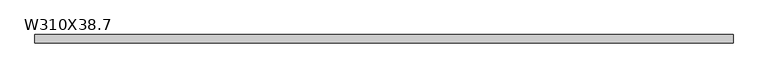
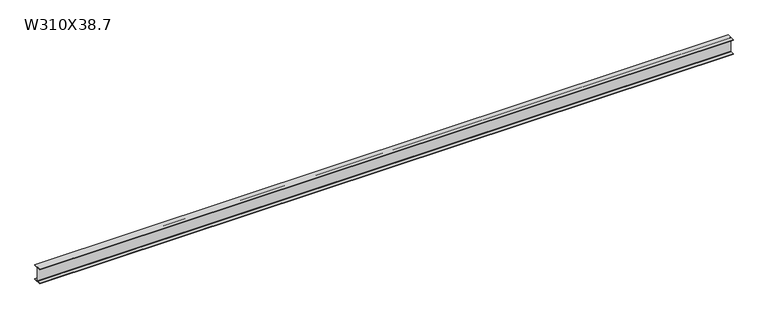
"""IFC4 building model written with IfcOpenShell, lengths in millimetres: beam geometry, M_W Shapes : W310X38.7."""

from ifc_helpers import new_model, si_unit, point, frame, frame_2d, origin, place, context, project, spatial, polyline, circle_curve, trimmed, segment, composite_curve, outline, extrude, source, transform, mapped, element, save


def w310x38_7_490d0887(model_context):
    return source(origin(), model_context, "Body", "SweptSolid", [
        extrude(outline(composite_curve([segment(polyline([(82.5, -145.35), (82.5, -155.0), (-82.5, -155.0), (-82.5, -145.35), (-10.57, -145.35)]), True, "CONTINUOUS"), segment(trimmed(circle_curve(frame_2d((-10.57, -137.7)), 7.65), [point((-10.57, -145.35))], [point((-2.92, -137.7))], True, "CARTESIAN"), True, "CONTINUOUS"), segment(polyline([(-2.92, -137.7), (-2.92, 137.7)]), True, "CONTINUOUS"), segment(trimmed(circle_curve(frame_2d((-10.57, 137.7)), 7.65), [point((-2.92, 137.7))], [point((-10.57, 145.35))], True, "CARTESIAN"), True, "CONTINUOUS"), segment(polyline([(-10.57, 145.35), (-82.5, 145.35), (-82.5, 155.0), (82.5, 155.0), (82.5, 145.35), (10.57, 145.35)]), True, "CONTINUOUS"), segment(trimmed(circle_curve(frame_2d((10.57, 137.7)), 7.65), [point((10.57, 145.35))], [point((2.92, 137.7))], True, "CARTESIAN"), True, "CONTINUOUS"), segment(polyline([(2.92, 137.7), (2.92, -137.7)]), True, "CONTINUOUS"), segment(trimmed(circle_curve(frame_2d((10.57, -137.7)), 7.65), [point((2.92, -137.7))], [point((10.57, -145.35))], True, "CARTESIAN"), True, "CONTINUOUS"), segment(polyline([(10.57, -145.35), (82.5, -145.35)]), True, "CONTINUOUS")], self_intersect=False)), frame((-6823.05, 0.0, 0.0), z_axis=(1.0, 0.0, 0.0), x_axis=(0.0, 1.0, 0.0)), (0.0, 0.0, 1.0), 14024.0),
    ])


if __name__ == "__main__":
    model = new_model("IFC4")
    model_context = context("Model", 3, world=origin())
    ifc_project = project(units=[si_unit("LENGTHUNIT", "METRE", prefix="MILLI")], contexts=[model_context])
    site = spatial("IfcSite", under=ifc_project)
    building = spatial("IfcBuilding", under=site)
    placement = place(None, origin())
    w310x38_7_shape = w310x38_7_490d0887(model_context)
    element("IfcBeam", 1, ObjectType="M_W Shapes : W310X38.7", at=placement, inside=building, context=model_context, shape_type="MappedRepresentation", body=[
        mapped(w310x38_7_shape, transform((0.0, 0.0, 0.0), x_axis=(1.0, 0.0, 0.0), y_axis=(0.0, 1.0, 0.0), z_axis=(0.0, 0.0, 1.0))),
    ])
    save(model, "model.ifc")

# Revit data of these elements
# Type "M_W Shapes : W310X38.7"
#   Section Name Key = "W12x26"
#   Width = 165 mm
#   Web Thickness = 5.84 mm
#   Web Fillet = 7.65 mm
#   Warping Constant = 163000 cm⁶
#   Torsional Moment of Inertia = 12.5 cm⁴
#   Section Area = 49.4 cm²
#   Plastic Modulus weak axis = 0.00473217 (stored number, unit not read)
#   Plastic Modulus strong axis = 0.0215419 (stored number, unit not read)
#   Perimeter = 1.25 m²/m
#   Nominal Weight = 379.516 N/m
#   Moment of Inertia weak axis = 720 cm⁴
#   Moment of Inertia strong axis = 8490 cm⁴
#   Height = 310 mm
#   Flange Thickness = 9.65 mm
#   Elastic Modulus weak axis = 0.00309003 (stored number, unit not read)
#   Elastic Modulus strong axis = 0.0193171 (stored number, unit not read)
#   Centroid Vertical = 155 mm
#   Centroid Horizontal = 82.5 mm
#   Length [instance default] = 1.5 m
#   Structural Material [instance default] = Steel, 45-345
#   Assembly Code = ""
# Element 1 (IfcBeam, "M_W Shapes : W310X38.7")
#   Materials on its faces: "Steel, 45-345"
# Materials
#   "Steel, 45-345": class "Metal", colour RGB 189 187 185, transparency 0, Description = "Steel 345 MPa", Cost = 0
